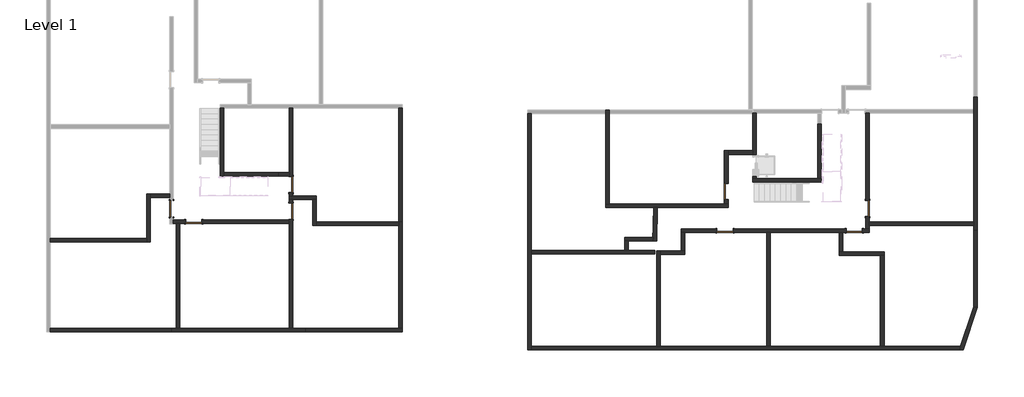
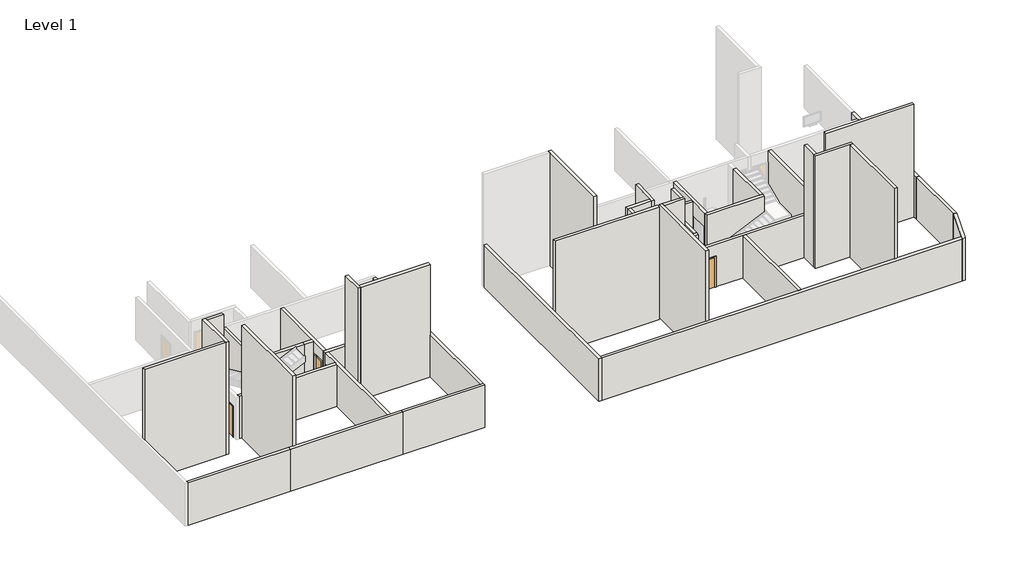
# One storey, part 1 of 2: 44 walls, 8 doors.
"""IFC4 building model written with IfcOpenShell, lengths in millimetres."""

import ifcopenshell
import ifcopenshell.guid

model = None  # the IFC model being written
_history = None  # IfcOwnerHistory: only IFC2X3 demands one
_inside = {}  # id of a spatial element -> (the spatial element, [elements in it])
_under = {}  # id of a project, library or spatial element -> (it, [spatial elements below it])
_declared = {}  # id of a project -> (the project, [libraries it declares])
_typed = {}  # id of a type object -> (the type object, [elements of that type])
_made_of = {}  # id of a material, layer set ... -> (it, [elements and type objects made of it])


def new_model(schema):
    """Start an empty IFC model of exactly this schema.

    Asked for "IFC4X3", IfcOpenShell would pick the latest addendum, in which some entities
    have other attributes; the version numbers below select the first issue.
    IFC2X3 requires an IfcOwnerHistory on every rooted entity: one is made here for all.
    """
    global model, _history
    if schema == "IFC4X3":
        model = ifcopenshell.file(schema_version=(4, 3, 0, 0))
    else:
        model = ifcopenshell.file(schema=schema)
    _inside.clear()
    _under.clear()
    _declared.clear()
    _typed.clear()
    _made_of.clear()
    _history = None
    if model.schema == "IFC2X3":
        org = make("IfcOrganization", Name="unknown")
        user = make(
            "IfcPersonAndOrganization",
            ThePerson=make("IfcPerson", FamilyName="unknown"),
            TheOrganization=org,
        )
        app = make(
            "IfcApplication",
            ApplicationDeveloper=org,
            Version="unknown",
            ApplicationFullName="unknown",
            ApplicationIdentifier="unknown",
        )
        _history = make(
            "IfcOwnerHistory",
            OwningUser=user,
            OwningApplication=app,
            ChangeAction="ADDED",
            CreationDate=0,
        )
    return model


def make(cls, **values):
    """One entity of the class cls with the attributes given. An attribute that is None is left unset."""
    return model.create_entity(
        cls, **{name: value for name, value in values.items() if value is not None}
    )


def rooted(cls, **values):
    """An entity with a GlobalId (a new one), such as an element, a storey or a relation."""
    return make(cls, GlobalId=ifcopenshell.guid.new(), OwnerHistory=_history, **values)


def si_unit(unit_type, name, prefix=None):
    """IfcSIUnit, for example si_unit("LENGTHUNIT", "METRE", prefix="MILLI")."""
    return make("IfcSIUnit", UnitType=unit_type, Prefix=prefix, Name=name)


def assignment(units):
    """IfcUnitAssignment: the units of a project."""
    return None if units is None else make("IfcUnitAssignment", Units=units)


def point(xyz):
    """IfcCartesianPoint."""
    return None if xyz is None else make("IfcCartesianPoint", Coordinates=xyz)


def direction(xyz):
    """IfcDirection."""
    return None if xyz is None else make("IfcDirection", DirectionRatios=xyz)


def frame(location, z_axis=None, x_axis=None):
    """IfcAxis2Placement3D, a coordinate frame: its origin and axes. An axis left out is left unset."""
    return make(
        "IfcAxis2Placement3D",
        Location=point(location),
        Axis=direction(z_axis),
        RefDirection=direction(x_axis),
    )


def origin():
    """The frame at (0, 0, 0) with its axes left unset."""
    return frame((0.0, 0.0, 0.0))


def origin_with_axes():
    """The frame at (0, 0, 0) with the z axis (0, 0, 1) and the x axis (1, 0, 0) written out."""
    return frame((0.0, 0.0, 0.0), z_axis=(0.0, 0.0, 1.0), x_axis=(1.0, 0.0, 0.0))


def place(relative_to, where):
    """IfcLocalPlacement: puts the frame where relative to a parent placement (None: the world)."""
    return make(
        "IfcLocalPlacement", PlacementRelTo=relative_to, RelativePlacement=where
    )


def context(
    kind, dimensions, precision=None, world=None, true_north=None, identifier=None
):
    """IfcGeometricRepresentationContext, for example the 3D "Model" context."""
    return make(
        "IfcGeometricRepresentationContext",
        ContextIdentifier=identifier,
        ContextType=kind,
        CoordinateSpaceDimension=dimensions,
        Precision=precision,
        WorldCoordinateSystem=world,
        TrueNorth=true_north,
    )


def project(units=None, contexts=None):
    """IfcProject with its units and contexts."""
    return rooted(
        "IfcProject",
        Name="project",
        RepresentationContexts=contexts,
        UnitsInContext=assignment(units),
    )


def spatial(cls, under=None, at=None, **own):
    """A site, building, storey or space (cls), placed at a placement, below another one or the project."""
    s = rooted(cls, ObjectPlacement=at, **own)
    if under is not None:
        _under.setdefault(under.id(), (under, []))[1].append(s)
    return s


def polyline(points):
    """IfcPolyline through the points."""
    return make("IfcPolyline", Points=[point(p) for p in points])


def outline(outer, holes=None, kind="AREA"):
    """IfcArbitraryClosedProfileDef: a profile drawn as a closed curve; with holes, ...WithVoids."""
    if holes is None:
        return make("IfcArbitraryClosedProfileDef", ProfileType=kind, OuterCurve=outer)
    return make(
        "IfcArbitraryProfileDefWithVoids",
        ProfileType=kind,
        OuterCurve=outer,
        InnerCurves=holes,
    )


def extrude(swept, where, along, depth):
    """IfcExtrudedAreaSolid: the profile swept, set in the frame where, extruded along a direction by depth."""
    return make(
        "IfcExtrudedAreaSolid",
        SweptArea=swept,
        Position=where,
        ExtrudedDirection=direction(along),
        Depth=depth,
    )


def faces_of(points, faces, orient=None, outer=None):
    """IfcFace entities. A face is a list of loops; a loop is a list of indices into points, from 0.

    orient and outer hold one flag for each loop. By default every Orientation is true, the
    first loop of a face is its IfcFaceOuterBound and the others are IfcFaceBound.
    """
    made = []
    for i, loops in enumerate(faces):
        bounds = []
        for j, loop in enumerate(loops):
            is_outer = j == 0 if outer is None else outer[i][j]
            bounds.append(
                make(
                    "IfcFaceOuterBound" if is_outer else "IfcFaceBound",
                    Bound=make("IfcPolyLoop", Polygon=[points[k] for k in loop]),
                    Orientation=True if orient is None else orient[i][j],
                )
            )
        made.append(make("IfcFace", Bounds=bounds))
    return made


def faceted_brep(points, faces, orient=None, outer=None, voids=None):
    """IfcFacetedBrep: a solid bounded by flat faces; with voids (closed shells), ...WithVoids."""
    shared = [point(p) for p in points]
    hull = make("IfcClosedShell", CfsFaces=faces_of(shared, faces, orient, outer))
    if voids is None:
        return make("IfcFacetedBrep", Outer=hull)
    return make(
        "IfcFacetedBrepWithVoids",
        Outer=hull,
        Voids=[
            make(cls, CfsFaces=faces_of(shared, fs, o, b)) for cls, fs, o, b in voids
        ],
    )


def shape(context_of_items, identifier, shape_type, items):
    """IfcShapeRepresentation: the items that make up one representation, for example the "Body"."""
    return make(
        "IfcShapeRepresentation",
        ContextOfItems=context_of_items,
        RepresentationIdentifier=identifier,
        RepresentationType=shape_type,
        Items=items,
    )


def source(mapping_origin, context_of_items, identifier, shape_type, items):
    """IfcRepresentationMap: a shape defined once, which mapped items show again and again."""
    return make(
        "IfcRepresentationMap",
        MappingOrigin=mapping_origin,
        MappedRepresentation=shape(context_of_items, identifier, shape_type, items),
    )


def transform(
    local_origin,
    x_axis=None,
    y_axis=None,
    z_axis=None,
    scale=None,
    scale2=None,
    scale3=None,
    uniform=True,
):
    """IfcCartesianTransformationOperator3D, or its non-uniform kind. x_axis, y_axis, z_axis: its Axis1, 2, 3."""
    if uniform:
        return make(
            "IfcCartesianTransformationOperator3D",
            Axis1=direction(x_axis),
            Axis2=direction(y_axis),
            LocalOrigin=point(local_origin),
            Scale=scale,
            Axis3=direction(z_axis),
        )
    return make(
        "IfcCartesianTransformationOperator3DnonUniform",
        Axis1=direction(x_axis),
        Axis2=direction(y_axis),
        LocalOrigin=point(local_origin),
        Scale=scale,
        Axis3=direction(z_axis),
        Scale2=scale2,
        Scale3=scale3,
    )


def mapped(mapping_source, mapping_target):
    """IfcMappedItem: shows the shape of a source again, moved by a transform."""
    return make(
        "IfcMappedItem", MappingSource=mapping_source, MappingTarget=mapping_target
    )


def made_of(thing, what):
    """Note that an element or type object is made of a material, layer set ...; save() writes the relation."""
    if what is not None:
        _made_of.setdefault(what.id(), (what, []))[1].append(thing)
    return thing


def element(
    cls,
    number,
    at=None,
    inside=None,
    cuts=None,
    type_object=None,
    material=None,
    context=None,
    identifier="Body",
    shape_type=None,
    held_by="IfcProductDefinitionShape",
    body=None,
    shapes=None,
    **own,
):
    """One element of the class cls, such as IfcWall. Its Tag is "e" and its number.

    at: its placement. inside: the storey or other place that contains it. cuts: it is an
    opening in that element (IfcRelVoidsElement). A single representation is given by context,
    identifier, shape_type and body (its items); several are given by shapes. held_by: the class
    of the entity that holds the representations. save() writes the other relations.
    """
    e = rooted(cls, Tag="e%d" % number, ObjectPlacement=at, **own)
    if body is not None:
        shapes = [shape(context, identifier, shape_type, body)]
    if shapes is not None:
        e.Representation = make(held_by, Representations=shapes)
    if inside is not None:
        _inside.setdefault(inside.id(), (inside, []))[1].append(e)
    if cuts is not None:
        rooted(
            "IfcRelVoidsElement", RelatingBuildingElement=cuts, RelatedOpeningElement=e
        )
    if type_object is not None:
        _typed.setdefault(type_object.id(), (type_object, []))[1].append(e)
    return made_of(e, material)


def aggregate(whole, parts):
    """IfcRelAggregates: a whole, such as a stair, and the parts it consists of."""
    return rooted("IfcRelAggregates", RelatingObject=whole, RelatedObjects=parts)


def save(model, path):
    """Write the relations noted so far, then the file.

    IfcRelAggregates (storeys below a building ...), IfcRelContainedInSpatialStructure (elements
    in a storey), IfcRelDefinesByType, IfcRelAssociatesMaterial and IfcRelDeclares: one each for
    every whole, place, type object, material and project.
    """
    for whole, parts in _under.values():
        aggregate(whole, parts)
    for where, things in _inside.values():
        rooted(
            "IfcRelContainedInSpatialStructure",
            RelatedElements=things,
            RelatingStructure=where,
        )
    for kind, things in _typed.values():
        rooted("IfcRelDefinesByType", RelatedObjects=things, RelatingType=kind)
    for what, things in _made_of.values():
        rooted("IfcRelAssociatesMaterial", RelatedObjects=things, RelatingMaterial=what)
    for by, libraries in _declared.values():
        rooted("IfcRelDeclares", RelatingContext=by, RelatedDefinitions=libraries)
    model.write(path)


def m_single_flush_0915_x_2134mm_727434cd(model_context):
    return source(origin(), model_context, "Body", "SweptSolid", [
        extrude(outline(polyline([(2210.0, -533.5), (0.0, -533.5), (0.0, -457.5), (2134.0, -457.5), (2134.0, 457.5), (0.0, 457.5), (0.0, 533.5), (2210.0, 533.5), (2210.0, -533.5)])), frame((0.0, -125.0, 0.0), z_axis=(0.0, 1.0, 0.0), x_axis=(0.0, 0.0, 1.0)), (0.0, 0.0, 1.0), 25.0),
        extrude(outline(polyline([(2210.0, 533.5), (2210.0, -533.5), (0.0, -533.5), (0.0, -457.5), (2134.0, -457.5), (2134.0, 457.5), (0.0, 457.5), (0.0, 533.5), (2210.0, 533.5)])), frame((0.0, 100.0, 0.0), z_axis=(0.0, 1.0, 0.0), x_axis=(0.0, 0.0, 1.0)), (0.0, 0.0, 1.0), 25.0),
        extrude(outline(polyline([(457.5, -49.0), (457.5, -100.0), (-457.5, -100.0), (-457.5, -49.0), (457.5, -49.0)])), origin_with_axes(), (0.0, 0.0, 1.0), 2134.0),
    ])


def m_single_flush_0915_x_2134mm_6a9e8738(model_context):
    return source(origin(), model_context, "Body", "SweptSolid", [
        extrude(outline(polyline([(2210.0, -533.5), (0.0, -533.5), (0.0, -457.5), (2134.0, -457.5), (2134.0, 457.5), (0.0, 457.5), (0.0, 533.5), (2210.0, 533.5), (2210.0, -533.5)])), frame((0.0, 100.0, 0.0), z_axis=(0.0, 1.0, 0.0), x_axis=(0.0, 0.0, 1.0)), (0.0, 0.0, 1.0), 25.0),
        extrude(outline(polyline([(2210.0, 533.5), (2210.0, -533.5), (0.0, -533.5), (0.0, -457.5), (2134.0, -457.5), (2134.0, 457.5), (0.0, 457.5), (0.0, 533.5), (2210.0, 533.5)])), frame((0.0, -125.0, 0.0), z_axis=(0.0, 1.0, 0.0), x_axis=(0.0, 0.0, 1.0)), (0.0, 0.0, 1.0), 25.0),
        extrude(outline(polyline([(457.5, 49.0), (-457.5, 49.0), (-457.5, 100.0), (457.5, 100.0), (457.5, 49.0)])), origin_with_axes(), (0.0, 0.0, 1.0), 2134.0),
    ])


model = new_model("IFC4")

# Units and contexts
model_context = context("Model", 3, world=origin())
ifc_project = project(units=[si_unit("LENGTHUNIT", "METRE", prefix="MILLI")], contexts=[model_context])

# Site, building, storey
site = spatial("IfcSite", under=ifc_project)
building = spatial("IfcBuilding", under=site)
storey = spatial("IfcBuildingStorey", under=building, Name="Level 1", Elevation=0.0)

# Doors
placement = place(None, origin())
m_single_flush_0915_x_2134mm_shape = m_single_flush_0915_x_2134mm_727434cd(model_context)
element("IfcDoor", 1, ObjectType="M_Single-Flush : 0915 x 2134mm", at=placement, inside=storey, context=model_context, shape_type="MappedRepresentation", body=[
    mapped(m_single_flush_0915_x_2134mm_shape, transform((16070.6041014, -3023.024372, 0.0), x_axis=(0.0, -1.0, 0.0), y_axis=(1.0, 0.0, 0.0), z_axis=(0.0, 0.0, 1.0))),
])
element("IfcDoor", 2, ObjectType="M_Single-Flush : 0915 x 2134mm", at=placement, inside=storey, context=model_context, shape_type="MappedRepresentation", body=[
    mapped(m_single_flush_0915_x_2134mm_shape, transform((16002.336337, -5240.0098119, 0.0), x_axis=(1.0, 0.0, 0.0), y_axis=(0.0, 1.0, 0.0), z_axis=(0.0, 0.0, 1.0))),
])
element("IfcDoor", 3, ObjectType="M_Single-Flush : 0915 x 2134mm", at=placement, inside=storey, context=model_context, shape_type="MappedRepresentation", body=[
    mapped(m_single_flush_0915_x_2134mm_shape, transform((-8530.3449834, -4137.6378151, 0.0), x_axis=(0.0, 1.0, 0.0), y_axis=(-1.0, 0.0, 0.0), z_axis=(0.0, 0.0, 1.0))),
])
m_single_flush_0915_x_2134mm_2_shape = m_single_flush_0915_x_2134mm_6a9e8738(model_context)
element("IfcDoor", 4, ObjectType="M_Single-Flush : 0915 x 2134mm", at=placement, inside=storey, context=model_context, shape_type="MappedRepresentation", body=[
    mapped(m_single_flush_0915_x_2134mm_2_shape, transform((24048.8612349, -3982.5098119, 0.0), x_axis=(0.0, -1.0, 0.0), y_axis=(1.0, 0.0, 0.0), z_axis=(0.0, 0.0, 1.0))),
])
element("IfcDoor", 5, ObjectType="M_Single-Flush : 0915 x 2134mm", at=placement, inside=storey, context=model_context, shape_type="MappedRepresentation", body=[
    mapped(m_single_flush_0915_x_2134mm_2_shape, transform((23308.8612349, -5240.0098119, 0.0), x_axis=(-1.0, 0.0, 0.0), y_axis=(0.0, -1.0, 0.0), z_axis=(0.0, 0.0, 1.0))),
])
element("IfcDoor", 6, ObjectType="M_Single-Flush : 0915 x 2134mm", at=placement, inside=storey, context=model_context, shape_type="MappedRepresentation", body=[
    mapped(m_single_flush_0915_x_2134mm_2_shape, transform((-14032.3304233, -4739.1627129, 0.0), x_axis=(-1.0, 0.0, 0.0), y_axis=(0.0, -1.0, 0.0), z_axis=(0.0, 0.0, 1.0))),
])
element("IfcDoor", 7, ObjectType="M_Single-Flush : 0915 x 2134mm", at=placement, inside=storey, context=model_context, shape_type="MappedRepresentation", body=[
    mapped(m_single_flush_0915_x_2134mm_2_shape, transform((-8530.3449834, -2622.6378151, 0.0), x_axis=(0.0, -1.0, 0.0), y_axis=(1.0, 0.0, 0.0), z_axis=(0.0, 0.0, 1.0))),
])
element("IfcDoor", 8, ObjectType="M_Single-Flush : 0915 x 2134mm", at=placement, inside=storey, context=model_context, shape_type="MappedRepresentation", body=[
    mapped(m_single_flush_0915_x_2134mm_2_shape, transform((-15289.8304233, -3999.1627129, 0.0), x_axis=(0.0, 1.0, 0.0), y_axis=(-1.0, 0.0, 0.0), z_axis=(0.0, 0.0, 1.0))),
])

# Walls
element("IfcWall", 9, ObjectType="Generic - 200mm", at=placement, inside=storey, context=model_context, shape_type="Brep", body=[
    faceted_brep([(30068.8612349, 2319.475628, 0.0), (30068.8612349, 1619.475628, 0.0), (30068.8612349, 1419.475628, 0.0), (30068.8612349, -4760.0098119, 0.0), (30068.8612349, -4960.0098119, 0.0), (30068.8612349, -5240.0098119, 0.0), (30068.8612349, -5240.0098119, 3000.0), (30068.8612349, 1419.475628, 3000.0), (30068.8612349, 1619.475628, 3000.0), (30068.8612349, 2319.475628, 3000.0), (30268.8612349, 2319.475628, 0.0), (30268.8612349, 2319.475628, 3000.0), (30268.8612349, -5240.0098119, 3000.0), (30268.8612349, -5240.0098119, 0.0), (30268.3425199, 2319.475628, 0.0), (30069.3799498, -5240.0098119, 0.0), (30069.3799498, -5240.0098119, 3000.0), (30268.3425199, 2319.475628, 3000.0)], [[[0, 1, 2, 3, 4, 5, 6, 7, 8, 9]], [[10, 11, 12, 13]], [[5, 4, 3, 2, 1, 0, 14, 10, 13, 15]], [[6, 5, 15, 13, 12, 16]], [[9, 8, 7, 6, 16, 12, 11, 17]], [[0, 9, 17, 11, 10, 14]]]),
])
element("IfcWall", 10, ObjectType="Generic - 200mm", at=placement, inside=storey, context=model_context, shape_type="Brep", body=[
    faceted_brep([(30069.3799498, -5240.0098119, 0.0), (30069.3799498, -9543.0251929, 0.0), (30069.3799498, -9543.0251929, 3000.0), (30069.3799498, -5240.0098119, 3000.0), (30269.3799498, -5240.0098119, 0.0), (30269.3799498, -5240.0098119, 3000.0), (30269.3799498, -9575.863443, 3000.0), (30269.3799498, -9575.863443, 0.0), (30268.8612349, -5240.0098119, 0.0), (30268.8612349, -5240.0098119, 3000.0)], [[[0, 1, 2, 3]], [[4, 5, 6, 7]], [[1, 0, 8, 4, 7]], [[3, 2, 6, 5, 9]], [[0, 3, 9, 5, 4, 8]], [[2, 1, 7, 6]]]),
])
element("IfcWall", 11, ObjectType="Generic - 200mm", at=placement, inside=storey, context=model_context, shape_type="Brep", body=[
    faceted_brep([(21449.836337, -2276.2808257, 0.0), (21249.836337, -2276.2808257, 0.0), (17770.6041014, -2276.2808257, 0.0), (17570.6041014, -2276.2808257, 0.0), (17570.6041014, -2276.2808257, 3000.0), (17770.6041014, -2276.2808257, 3000.0), (21249.836337, -2276.2808257, 3000.0), (21449.836337, -2276.2808257, 3000.0), (21449.836337, -2476.2808257, 0.0), (21449.836337, -2476.2808257, 3000.0), (17570.6041014, -2476.2808257, 3000.0), (17570.6041014, -2476.2808257, 0.0)], [[[0, 1, 2, 3, 4, 5, 6, 7]], [[8, 9, 10, 11]], [[3, 2, 1, 0, 8, 11]], [[7, 6, 5, 4, 10, 9]], [[0, 7, 9, 8]], [[4, 3, 11, 10]]]),
])
element("IfcWall", 12, ObjectType="Generic - 200mm", at=placement, inside=storey, context=model_context, shape_type="SweptSolid", body=[
    extrude(outline(polyline([(18559.836337, -5340.0098119), (18559.836337, -11796.6907835), (18359.836337, -11796.6907835), (18359.836337, -5340.0098119), (18559.836337, -5340.0098119)])), origin_with_axes(), (0.0, 0.0, 1.0), 3000.0),
])
element("IfcWall", 13, ObjectType="Generic - 200mm", at=placement, inside=storey, context=model_context, shape_type="Brep", body=[
    faceted_brep([(29308.8116245, -11796.6907835, 0.0), (24988.8612349, -11796.6907835, 0.0), (24788.8612349, -11796.6907835, 0.0), (18559.836337, -11796.6907835, 0.0), (18359.836337, -11796.6907835, 0.0), (12342.1281129, -11796.6907835, 0.0), (12142.1281129, -11796.6907835, 0.0), (5043.716007, -11796.6907835, 0.0), (5043.716007, -11796.6907835, 3000.0), (18359.836337, -11796.6907835, 3000.0), (18559.836337, -11796.6907835, 3000.0), (29308.8116245, -11796.6907835, 3000.0), (29241.3155126, -11996.6907835, 0.0), (29241.3155126, -11996.6907835, 3000.0), (5043.716007, -11996.6907835, 3000.0), (5043.716007, -11996.6907835, 0.0)], [[[0, 1, 2, 3, 4, 5, 6, 7, 8, 9, 10, 11]], [[12, 13, 14, 15]], [[7, 6, 5, 4, 3, 2, 1, 0, 12, 15]], [[11, 10, 9, 8, 14, 13]], [[0, 11, 13, 12]], [[8, 7, 15, 14]]]),
])
element("IfcWall", 14, ObjectType="Generic - 200mm", at=placement, inside=storey, context=model_context, shape_type="Brep", body=[
    faceted_brep([(30069.3799498, -9543.0251929, 0.0), (29308.8116245, -11796.6907835, 0.0), (29241.3155126, -11996.6907835, 0.0), (29241.3155126, -11996.6907835, 3000.0), (29308.8116245, -11796.6907835, 3000.0), (30069.3799498, -9543.0251929, 3000.0), (30269.3799498, -9575.863443, 0.0), (30269.3799498, -9575.863443, 3000.0), (29452.3977836, -11996.6907835, 3000.0), (29452.3977836, -11996.6907835, 0.0)], [[[0, 1, 2, 3, 4, 5]], [[6, 7, 8, 9]], [[2, 1, 0, 6, 9]], [[5, 4, 3, 8, 7]], [[0, 5, 7, 6]], [[3, 2, 9, 8]]]),
])
element("IfcWall", 15, ObjectType="Generic - 200mm", at=placement, inside=storey, context=model_context, shape_type="Brep", body=[
    faceted_brep([(22851.3612349, -5140.0098119, 2134.0), (22851.3612349, -5140.0098119, 0.0), (16459.836337, -5140.0098119, 0.0), (16459.836337, -5140.0098119, 2134.0), (15544.836337, -5140.0098119, 2134.0), (15544.836337, -5140.0098119, 0.0), (13532.1281129, -5140.0098119, 0.0), (13532.1281129, -5140.0098119, 3000.0), (23948.8612349, -5140.0098119, 3000.0), (24148.8612349, -5140.0098119, 3000.0), (24163.3998354, -5140.0098119, 3000.0), (24163.3998354, -5140.0098119, 0.0), (24148.8612349, -5140.0098119, 0.0), (23948.8612349, -5140.0098119, 0.0), (23766.3612349, -5140.0098119, 0.0), (23766.3612349, -5140.0098119, 2134.0), (16459.836337, -5340.0098119, 0.0), (18359.836337, -5340.0098119, 0.0), (18559.836337, -5340.0098119, 0.0), (22468.8612349, -5340.0098119, 0.0), (22668.8612349, -5340.0098119, 0.0), (22851.3612349, -5340.0098119, 0.0), (22851.3612349, -5340.0098119, 2134.0), (23766.3612349, -5340.0098119, 2134.0), (23766.3612349, -5340.0098119, 0.0), (24163.3998354, -5340.0098119, 0.0), (24163.3998354, -5340.0098119, 3000.0), (18559.836337, -5340.0098119, 3000.0), (18359.836337, -5340.0098119, 3000.0), (13532.1281129, -5340.0098119, 3000.0), (13532.1281129, -5340.0098119, 0.0), (13732.1281129, -5340.0098119, 0.0), (15544.836337, -5340.0098119, 0.0), (15544.836337, -5340.0098119, 2134.0), (16459.836337, -5340.0098119, 2134.0)], [[[0, 1, 2, 3, 4, 5, 6, 7, 8, 9, 10, 11, 12, 13, 14, 15]], [[16, 17, 18, 19, 20, 21, 22, 23, 24, 25, 26, 27, 28, 29, 30, 31, 32, 33, 34]], [[2, 1, 21, 20, 19, 18, 17, 16]], [[14, 13, 12, 11, 25, 24]], [[30, 6, 5, 32, 31]], [[10, 9, 8, 7, 29, 28, 27, 26]], [[11, 10, 26, 25]], [[34, 3, 2, 16]], [[4, 33, 32, 5]], [[33, 4, 3, 34]], [[22, 21, 1, 0]], [[23, 22, 0, 15]], [[24, 23, 15, 14]], [[7, 6, 30, 29]]]),
])
element("IfcWall", 16, ObjectType="Generic - 200mm", at=placement, inside=storey, context=model_context, shape_type="Brep", body=[
    faceted_brep([(4843.716007, 1379.9901881, 0.0), (4843.716007, -11996.6907835, 0.0), (4843.716007, -11996.6907835, 3000.0), (4843.716007, 1379.9901881, 3000.0), (5043.716007, 1379.9901881, 0.0), (5043.716007, 1379.9901881, 3000.0), (5043.716007, -11796.6907835, 3000.0), (5043.716007, -11996.6907835, 3000.0), (5043.716007, -11996.6907835, 0.0), (5043.716007, -11796.6907835, 0.0), (5043.716007, -6560.0098119, 0.0), (5043.716007, -6360.0098119, 0.0)], [[[0, 1, 2, 3]], [[4, 5, 6, 7, 8, 9, 10, 11]], [[1, 0, 4, 11, 10, 9, 8]], [[3, 2, 7, 6, 5]], [[2, 1, 8, 7]], [[0, 3, 5, 4]]]),
])
element("IfcWall", 17, ObjectType="Generic - 200mm", at=placement, inside=storey, context=model_context, shape_type="Brep", body=[
    faceted_brep([(24148.8612349, 1419.475628, 3000.0), (24148.8612349, -5140.0098119, 3000.0), (24148.8612349, -5140.0098119, 0.0), (24148.8612349, -4960.0098119, 0.0), (24148.8612349, -4760.0098119, 0.0), (24148.8612349, -4440.0098119, 0.0), (24148.8612349, -4440.0098119, 2134.0), (24148.8612349, -3525.0098119, 2134.0), (24148.8612349, -3525.0098119, 0.0), (24148.8612349, 1419.475628, 0.0), (23948.8612349, -5140.0098119, 3000.0), (23948.8612349, 1419.475628, 3000.0), (23948.8612349, 1419.475628, 0.0), (23948.8612349, -3525.0098119, 0.0), (23948.8612349, -3525.0098119, 2134.0), (23948.8612349, -4440.0098119, 2134.0), (23948.8612349, -4440.0098119, 0.0), (23948.8612349, -5140.0098119, 0.0)], [[[0, 1, 2, 3, 4, 5, 6, 7, 8, 9]], [[10, 11, 12, 13, 14, 15, 16, 17]], [[12, 9, 8, 13]], [[2, 17, 16, 5, 4, 3]], [[1, 0, 11, 10]], [[0, 9, 12, 11]], [[15, 6, 5, 16]], [[7, 14, 13, 8]], [[14, 7, 6, 15]], [[2, 1, 10, 17]]]),
])
element("IfcWall", 18, ObjectType="Generic - 200mm", at=placement, inside=storey, context=model_context, shape_type="SweptSolid", body=[
    extrude(outline(polyline([(21249.836337, -2276.2808257), (21249.836337, 799.475628), (21449.836337, 799.475628), (21449.836337, -2276.2808257), (21249.836337, -2276.2808257)])), origin_with_axes(), (0.0, 0.0, 1.0), 3000.0),
])
element("IfcWall", 19, ObjectType="Generic - 200mm", at=placement, inside=storey, context=model_context, shape_type="Brep", body=[
    faceted_brep([(17570.6041014, -2276.2808257, 3000.0), (17570.6041014, -920.524372, 3000.0), (17570.6041014, -720.524372, 3000.0), (17570.6041014, 1379.475628, 3000.0), (17570.6041014, 1419.475628, 3000.0), (17570.6041014, 1419.475628, 0.0), (17570.6041014, 1379.475628, 0.0), (17570.6041014, -720.524372, 0.0), (17570.6041014, -920.524372, 0.0), (17570.6041014, -926.2808257, 0.0), (17570.6041014, -926.2808257, 2000.0), (17570.6041014, -2181.2876228, 2000.0), (17570.6041014, -2181.2876228, 0.0), (17570.6041014, -2276.2808257, 0.0), (17770.6041014, 1419.475628, 3000.0), (17770.6041014, -2276.2808257, 3000.0), (17770.6041014, -2276.2808257, 0.0), (17770.6041014, -2181.2876228, 0.0), (17770.6041014, -2181.2876228, 2000.0), (17770.6041014, -926.2808257, 2000.0), (17770.6041014, -926.2808257, 0.0), (17770.6041014, 1419.475628, 0.0)], [[[0, 1, 2, 3, 4, 5, 6, 7, 8, 9, 10, 11, 12, 13]], [[14, 15, 16, 17, 18, 19, 20, 21]], [[16, 13, 12, 17]], [[5, 21, 20, 9, 8, 7, 6]], [[4, 3, 2, 1, 0, 15, 14]], [[0, 13, 16, 15]], [[5, 4, 14, 21]], [[11, 18, 17, 12]], [[19, 10, 9, 20]], [[10, 19, 18, 11]]]),
])
element("IfcWall", 20, ObjectType="Generic - 200mm", at=placement, inside=storey, context=model_context, shape_type="Brep", body=[
    faceted_brep([(9268.8612349, -3940.0098119, 0.0), (11970.0065607, -3940.0098119, 0.0), (12170.0511873, -3940.0098119, 0.0), (16170.6041014, -3940.0098119, 0.0), (16170.6041014, -3940.0098119, 3000.0), (9268.8612349, -3940.0098119, 3000.0), (9268.8612349, -3740.0098119, 0.0), (9268.8612349, -3740.0098119, 3000.0), (15970.6041014, -3740.0098119, 3000.0), (16170.6041014, -3740.0098119, 3000.0), (16170.6041014, -3740.0098119, 0.0), (15970.6041014, -3740.0098119, 0.0), (9468.8612349, -3740.0098119, 0.0)], [[[0, 1, 2, 3, 4, 5]], [[6, 7, 8, 9, 10, 11, 12]], [[3, 2, 1, 0, 6, 12, 11, 10]], [[5, 4, 9, 8, 7]], [[4, 3, 10, 9]], [[0, 5, 7, 6]]]),
])
element("IfcWall", 21, ObjectType="Generic - 200mm", at=placement, inside=storey, context=model_context, shape_type="Brep", body=[
    faceted_brep([(16170.6041014, -720.524372, 3000.0), (16170.6041014, -920.524372, 3000.0), (16170.6041014, -3740.0098119, 3000.0), (16170.6041014, -3740.0098119, 0.0), (16170.6041014, -3480.524372, 0.0), (16170.6041014, -3480.524372, 2134.0), (16170.6041014, -2565.524372, 2134.0), (16170.6041014, -2565.524372, 0.0), (16170.6041014, -920.524372, 0.0), (16170.6041014, -720.524372, 0.0), (15970.6041014, -3740.0098119, 3000.0), (15970.6041014, -720.524372, 3000.0), (15970.6041014, -720.524372, 0.0), (15970.6041014, -2565.524372, 0.0), (15970.6041014, -2565.524372, 2134.0), (15970.6041014, -3480.524372, 2134.0), (15970.6041014, -3480.524372, 0.0), (15970.6041014, -3740.0098119, 0.0)], [[[0, 1, 2, 3, 4, 5, 6, 7, 8, 9]], [[10, 11, 12, 13, 14, 15, 16, 17]], [[3, 17, 16, 4]], [[12, 9, 8, 7, 13]], [[2, 1, 0, 11, 10]], [[3, 2, 10, 17]], [[0, 9, 12, 11]], [[15, 5, 4, 16]], [[6, 14, 13, 7]], [[14, 6, 5, 15]]]),
])
element("IfcWall", 22, ObjectType="Generic - 200mm", at=placement, inside=storey, context=model_context, shape_type="SweptSolid", body=[
    extrude(outline(polyline([(17570.6041014, -920.524372), (16170.6041014, -920.524372), (16170.6041014, -720.524372), (17570.6041014, -720.524372), (17570.6041014, -920.524372)])), origin_with_axes(), (0.0, 0.0, 1.0), 3000.0),
])
element("IfcWall", 23, ObjectType="Generic - 200mm", at=placement, inside=storey, context=model_context, shape_type="Brep", body=[
    faceted_brep([(22468.8612349, -6641.2808257, 0.0), (24788.8612349, -6641.2808257, 0.0), (24988.8612349, -6641.2808257, 0.0), (24988.8612349, -6641.2808257, 8000.0), (24788.8612349, -6641.2808257, 8000.0), (22468.8612349, -6641.2808257, 8000.0), (22468.8612349, -6441.2808257, 0.0), (22468.8612349, -6441.2808257, 8000.0), (22668.8612349, -6441.2808257, 8000.0), (24988.8612349, -6441.2808257, 8000.0), (24988.8612349, -6441.2808257, 0.0), (22668.8612349, -6441.2808257, 0.0)], [[[0, 1, 2, 3, 4, 5]], [[6, 7, 8, 9, 10, 11]], [[2, 1, 0, 6, 11, 10]], [[5, 4, 3, 9, 8, 7]], [[3, 2, 10, 9]], [[0, 5, 7, 6]]]),
])
element("IfcWall", 24, ObjectType="Generic - 200mm", at=placement, inside=storey, context=model_context, shape_type="SweptSolid", body=[
    extrude(outline(polyline([(24788.8612349, -11796.6907835), (24788.8612349, -6641.2808257), (24988.8612349, -6641.2808257), (24988.8612349, -11796.6907835), (24788.8612349, -11796.6907835)])), origin_with_axes(), (0.0, 0.0, 1.0), 8000.0),
])
element("IfcWall", 25, ObjectType="Generic - 200mm", at=placement, inside=storey, context=model_context, shape_type="SweptSolid", body=[
    extrude(outline(polyline([(22668.8612349, -5340.0098119), (22668.8612349, -6441.2808257), (22468.8612349, -6441.2808257), (22468.8612349, -5340.0098119), (22668.8612349, -5340.0098119)])), origin_with_axes(), (0.0, 0.0, 1.0), 8000.0),
])
element("IfcWall", 26, ObjectType="Generic - 200mm", at=placement, inside=storey, context=model_context, shape_type="SweptSolid", body=[
    extrude(outline(polyline([(30068.8612349, -4960.0098119), (24148.8612349, -4960.0098119), (24148.8612349, -4760.0098119), (30068.8612349, -4760.0098119), (30068.8612349, -4960.0098119)])), origin_with_axes(), (0.0, 0.0, 1.0), 8000.0),
])
element("IfcWall", 27, ObjectType="Generic - 200mm", at=placement, inside=storey, context=model_context, shape_type="Brep", body=[
    faceted_brep([(9268.8612349, 1579.9901881, 0.0), (9268.8612349, 1379.9901881, 0.0), (9268.8612349, -3740.0098119, 0.0), (9268.8612349, -3740.0098119, 3000.0), (9268.8612349, -3740.0098119, 8000.0), (9268.8612349, 1379.9901881, 8000.0), (9268.8612349, 1579.9901881, 8000.0), (9468.8612349, 1579.9901881, 0.0), (9468.8612349, 1579.9901881, 8000.0), (9468.8612349, -3740.0098119, 8000.0), (9468.8612349, -3740.0098119, 0.0), (9468.8612349, 1379.475628, 0.0), (9468.8612349, 1579.475628, 0.0)], [[[0, 1, 2, 3, 4, 5, 6]], [[7, 8, 9, 10, 11, 12]], [[2, 1, 0, 7, 12, 11, 10]], [[6, 5, 4, 9, 8]], [[4, 3, 2, 10, 9]], [[0, 6, 8, 7]]]),
])
element("IfcWall", 28, ObjectType="Generic - 200mm", at=placement, inside=storey, context=model_context, shape_type="Brep", body=[
    faceted_brep([(12016.7908757, -6360.0098119, 0.0), (10530.3209687, -6360.0098119, 0.0), (10330.3209687, -6360.0098119, 0.0), (5043.716007, -6360.0098119, 0.0), (5043.716007, -6360.0098119, 8000.0), (10330.3209687, -6360.0098119, 8000.0), (10530.3209687, -6360.0098119, 8000.0), (12016.7908757, -6360.0098119, 8000.0), (12016.7908757, -6560.0098119, 0.0), (12016.7908757, -6560.0098119, 8000.0), (5043.716007, -6560.0098119, 8000.0), (5043.716007, -6560.0098119, 0.0)], [[[0, 1, 2, 3, 4, 5, 6, 7]], [[8, 9, 10, 11]], [[3, 2, 1, 0, 8, 11]], [[7, 6, 5, 4, 10, 9]], [[0, 7, 9, 8]], [[4, 3, 11, 10]]]),
])
element("IfcWall", 29, ObjectType="Generic - 200mm", at=placement, inside=storey, context=model_context, shape_type="Brep", body=[
    faceted_brep([(-2430.3449834, -4740.1378151, 0.0), (-2430.3449834, -4940.1378151, 0.0), (-2430.3449834, -10758.643998, 0.0), (-2430.3449834, -10758.643998, 3000.0), (-2430.3449834, -4740.1378151, 3000.0), (-2230.3449834, -4740.1378151, 0.0), (-2230.3449834, -4740.1378151, 3000.0), (-2230.3449834, -10758.643998, 3000.0), (-2230.3449834, -10758.643998, 0.0)], [[[0, 1, 2, 3, 4]], [[5, 6, 7, 8]], [[2, 1, 0, 5, 8]], [[4, 3, 7, 6]], [[3, 2, 8, 7]], [[0, 4, 6, 5]]]),
])
element("IfcWall", 30, ObjectType="Generic - 200mm", at=placement, inside=storey, context=model_context, shape_type="Brep", body=[
    faceted_brep([(-2230.3449834, -10758.643998, 0.0), (-2430.3449834, -10758.643998, 0.0), (-7730.3449834, -10758.643998, 0.0), (-7730.3449834, -10758.643998, 3000.0), (-2430.3449834, -10758.643998, 3000.0), (-2230.3449834, -10758.643998, 3000.0), (-2230.3449834, -10958.643998, 0.0), (-2230.3449834, -10958.643998, 3000.0), (-7730.3449834, -10958.643998, 3000.0), (-7730.3449834, -10958.643998, 0.0), (-7730.3449834, -10759.1627129, 0.0), (-7730.3449834, -10759.1627129, 3000.0)], [[[0, 1, 2, 3, 4, 5]], [[6, 7, 8, 9]], [[2, 1, 0, 6, 9, 10]], [[3, 2, 10, 9, 8, 11]], [[5, 4, 3, 11, 8, 7]], [[0, 5, 7, 6]]]),
])
element("IfcWall", 31, ObjectType="Generic - 200mm", at=placement, inside=storey, context=model_context, shape_type="Brep", body=[
    faceted_brep([(-7730.3449834, -10759.1627129, 0.0), (-8430.3449834, -10759.1627129, 0.0), (-8630.3449834, -10759.1627129, 0.0), (-14809.8304233, -10759.1627129, 0.0), (-15009.8304233, -10759.1627129, 0.0), (-15289.8304233, -10759.1627129, 0.0), (-15289.8304233, -10759.1627129, 3000.0), (-8630.3449834, -10759.1627129, 3000.0), (-8430.3449834, -10759.1627129, 3000.0), (-7730.3449834, -10759.1627129, 3000.0), (-7730.3449834, -10959.1627129, 0.0), (-7730.3449834, -10959.1627129, 3000.0), (-15289.8304233, -10959.1627129, 3000.0), (-15289.8304233, -10959.1627129, 0.0), (-7730.3449834, -10958.643998, 0.0), (-15289.8304233, -10759.6814279, 0.0), (-15289.8304233, -10759.6814279, 3000.0), (-7730.3449834, -10958.643998, 3000.0)], [[[0, 1, 2, 3, 4, 5, 6, 7, 8, 9]], [[10, 11, 12, 13]], [[5, 4, 3, 2, 1, 0, 14, 10, 13, 15]], [[6, 5, 15, 13, 12, 16]], [[9, 8, 7, 6, 16, 12, 11, 17]], [[0, 9, 17, 11, 10, 14]]]),
])
element("IfcWall", 32, ObjectType="Generic - 200mm", at=placement, inside=storey, context=model_context, shape_type="Brep", body=[
    faceted_brep([(-15289.8304233, -10759.6814279, 0.0), (-22146.5113948, -10759.6814279, 0.0), (-22146.5113948, -10759.6814279, 3000.0), (-15289.8304233, -10759.6814279, 3000.0), (-15289.8304233, -10959.6814279, 0.0), (-15289.8304233, -10959.6814279, 3000.0), (-22146.5113948, -10959.6814279, 3000.0), (-22146.5113948, -10959.6814279, 0.0), (-15289.8304233, -10959.1627129, 0.0), (-15289.8304233, -10959.1627129, 3000.0)], [[[0, 1, 2, 3]], [[4, 5, 6, 7]], [[1, 0, 8, 4, 7]], [[3, 2, 6, 5, 9]], [[0, 3, 9, 5, 4, 8]], [[2, 1, 7, 6]]]),
])
element("IfcWall", 33, ObjectType="Generic - 200mm", at=placement, inside=storey, context=model_context, shape_type="Brep", body=[
    faceted_brep([(-12326.101437, -2140.1378151, 0.0), (-12326.101437, -1940.1378151, 0.0), (-12326.101437, 1699.0944206, 0.0), (-12326.101437, 1699.0944206, 3000.0), (-12326.101437, -1940.1378151, 3000.0), (-12326.101437, -2140.1378151, 3000.0), (-12526.101437, -2140.1378151, 0.0), (-12526.101437, -2140.1378151, 3000.0), (-12526.101437, 1699.0944206, 3000.0), (-12526.101437, 1699.0944206, 0.0)], [[[0, 1, 2, 3, 4, 5]], [[6, 7, 8, 9]], [[2, 1, 0, 6, 9]], [[3, 2, 9, 8]], [[5, 4, 3, 8, 7]], [[0, 5, 7, 6]]]),
])
element("IfcWall", 34, ObjectType="Generic - 200mm", at=placement, inside=storey, context=model_context, shape_type="Brep", body=[
    faceted_brep([(-8630.3449834, -4839.1627129, 3000.0), (-15189.8304233, -4839.1627129, 3000.0), (-15189.8304233, -4839.1627129, 0.0), (-15009.8304233, -4839.1627129, 0.0), (-14809.8304233, -4839.1627129, 0.0), (-14489.8304233, -4839.1627129, 0.0), (-14489.8304233, -4839.1627129, 2134.0), (-13574.8304233, -4839.1627129, 2134.0), (-13574.8304233, -4839.1627129, 0.0), (-8630.3449834, -4839.1627129, 0.0), (-15189.8304233, -4639.1627129, 3000.0), (-8630.3449834, -4639.1627129, 3000.0), (-8630.3449834, -4639.1627129, 0.0), (-13574.8304233, -4639.1627129, 0.0), (-13574.8304233, -4639.1627129, 2134.0), (-14489.8304233, -4639.1627129, 2134.0), (-14489.8304233, -4639.1627129, 0.0), (-15189.8304233, -4639.1627129, 0.0)], [[[0, 1, 2, 3, 4, 5, 6, 7, 8, 9]], [[10, 11, 12, 13, 14, 15, 16, 17]], [[12, 9, 8, 13]], [[2, 17, 16, 5, 4, 3]], [[1, 0, 11, 10]], [[0, 9, 12, 11]], [[15, 6, 5, 16]], [[7, 14, 13, 8]], [[14, 7, 6, 15]], [[2, 1, 10, 17]]]),
])
element("IfcWall", 35, ObjectType="Generic - 200mm", at=placement, inside=storey, context=model_context, shape_type="SweptSolid", body=[
    extrude(outline(polyline([(-12326.101437, -1940.1378151), (-9250.3449834, -1940.1378151), (-9250.3449834, -2140.1378151), (-12326.101437, -2140.1378151), (-12326.101437, -1940.1378151)])), origin_with_axes(), (0.0, 0.0, 1.0), 3000.0),
])
element("IfcWall", 36, ObjectType="Generic - 200mm", at=placement, inside=storey, context=model_context, shape_type="SweptSolid", body=[
    extrude(outline(polyline([(-8630.3449834, -2140.1378151), (-9250.3449834, -2140.1378151), (-9250.3449834, -1940.1378151), (-8630.3449834, -1940.1378151), (-8630.3449834, -2140.1378151)])), origin_with_axes(), (0.0, 0.0, 1.0), 3000.0),
])
element("IfcWall", 37, ObjectType="Generic - 200mm", at=placement, inside=storey, context=model_context, shape_type="SweptSolid", body=[
    extrude(outline(polyline([(-2430.3449834, -4740.1378151), (-2430.3449834, 1700.8372871), (-2230.3449834, 1700.8372871), (-2230.3449834, -4740.1378151), (-2430.3449834, -4740.1378151)])), origin_with_axes(), (0.0, 0.0, 1.0), 3000.0),
])
element("IfcWall", 38, ObjectType="Generic - 200mm", at=placement, inside=storey, context=model_context, shape_type="Brep", body=[
    faceted_brep([(-8630.3449834, -3480.1378151, 0.0), (-8430.3449834, -3480.1378151, 0.0), (-7295.3449834, -3480.1378151, 0.0), (-7095.3449834, -3480.1378151, 0.0), (-7095.3449834, -3480.1378151, 3000.0), (-8430.3449834, -3480.1378151, 3000.0), (-8630.3449834, -3480.1378151, 3000.0), (-8630.3449834, -3280.1378151, 0.0), (-8630.3449834, -3280.1378151, 3000.0), (-8430.3449834, -3280.1378151, 3000.0), (-7095.3449834, -3280.1378151, 3000.0), (-7095.3449834, -3280.1378151, 0.0), (-8430.3449834, -3280.1378151, 0.0)], [[[0, 1, 2, 3, 4, 5, 6]], [[7, 8, 9, 10, 11, 12]], [[3, 2, 1, 0, 7, 12, 11]], [[6, 5, 4, 10, 9, 8]], [[0, 6, 8, 7]], [[4, 3, 11, 10]]]),
])
element("IfcWall", 39, ObjectType="Generic - 200mm", at=placement, inside=storey, context=model_context, shape_type="Brep", body=[
    faceted_brep([(-8630.3449834, -10759.1627129, 3000.0), (-8630.3449834, -4839.1627129, 3000.0), (-8630.3449834, -4639.1627129, 3000.0), (-8630.3449834, -3480.1378151, 3000.0), (-8630.3449834, -3480.1378151, 0.0), (-8630.3449834, -3680.1378151, 0.0), (-8630.3449834, -3680.1378151, 2134.0), (-8630.3449834, -4595.1378151, 2134.0), (-8630.3449834, -4595.1378151, 0.0), (-8630.3449834, -4639.1627129, 0.0), (-8630.3449834, -4839.1627129, 0.0), (-8630.3449834, -10759.1627129, 0.0), (-8430.3449834, -3480.1378151, 3000.0), (-8430.3449834, -10759.1627129, 3000.0), (-8430.3449834, -10759.1627129, 0.0), (-8430.3449834, -4595.1378151, 0.0), (-8430.3449834, -4595.1378151, 2134.0), (-8430.3449834, -3680.1378151, 2134.0), (-8430.3449834, -3680.1378151, 0.0), (-8430.3449834, -3480.1378151, 0.0)], [[[0, 1, 2, 3, 4, 5, 6, 7, 8, 9, 10, 11]], [[12, 13, 14, 15, 16, 17, 18, 19]], [[14, 11, 10, 9, 8, 15]], [[4, 19, 18, 5]], [[3, 2, 1, 0, 13, 12]], [[0, 11, 14, 13]], [[4, 3, 12, 19]], [[17, 6, 5, 18]], [[7, 16, 15, 8]], [[16, 7, 6, 17]]]),
])
element("IfcWall", 40, ObjectType="Generic - 200mm", at=placement, inside=storey, context=model_context, shape_type="Brep", body=[
    faceted_brep([(-8430.3449834, 1700.8372871, 3000.0), (-8430.3449834, -3280.1378151, 3000.0), (-8430.3449834, -3280.1378151, 0.0), (-8430.3449834, -3080.1378151, 0.0), (-8430.3449834, -3080.1378151, 2134.0), (-8430.3449834, -2165.1378151, 2134.0), (-8430.3449834, -2165.1378151, 0.0), (-8430.3449834, 1700.8372871, 0.0), (-8630.3449834, -3280.1378151, 3000.0), (-8630.3449834, -2140.1378151, 3000.0), (-8630.3449834, -1940.1378151, 3000.0), (-8630.3449834, 1700.8372871, 3000.0), (-8630.3449834, 1700.8372871, 0.0), (-8630.3449834, -1940.1378151, 0.0), (-8630.3449834, -2140.1378151, 0.0), (-8630.3449834, -2165.1378151, 0.0), (-8630.3449834, -2165.1378151, 2134.0), (-8630.3449834, -3080.1378151, 2134.0), (-8630.3449834, -3080.1378151, 0.0), (-8630.3449834, -3280.1378151, 0.0)], [[[0, 1, 2, 3, 4, 5, 6, 7]], [[8, 9, 10, 11, 12, 13, 14, 15, 16, 17, 18, 19]], [[2, 19, 18, 3]], [[12, 7, 6, 15, 14, 13]], [[1, 0, 11, 10, 9, 8]], [[2, 1, 8, 19]], [[17, 4, 3, 18]], [[5, 16, 15, 6]], [[16, 5, 4, 17]], [[0, 7, 12, 11]]]),
])
element("IfcWall", 41, ObjectType="Generic - 200mm", at=placement, inside=storey, context=model_context, shape_type="Brep", body=[
    faceted_brep([(-7295.3449834, -3480.1378151, 0.0), (-7295.3449834, -4940.1378151, 0.0), (-7295.3449834, -4940.1378151, 8000.0), (-7295.3449834, -3480.1378151, 8000.0), (-7095.3449834, -3480.1378151, 0.0), (-7095.3449834, -3480.1378151, 3000.0), (-7095.3449834, -3480.1378151, 8000.0), (-7095.3449834, -4740.1378151, 8000.0), (-7095.3449834, -4940.1378151, 8000.0), (-7095.3449834, -4940.1378151, 0.0), (-7095.3449834, -4740.1378151, 0.0)], [[[0, 1, 2, 3]], [[4, 5, 6, 7, 8, 9, 10]], [[1, 0, 4, 10, 9]], [[3, 2, 8, 7, 6]], [[2, 1, 9, 8]], [[0, 3, 6, 5, 4]]]),
])
element("IfcWall", 42, ObjectType="Generic - 200mm", at=placement, inside=storey, context=model_context, shape_type="Brep", body=[
    faceted_brep([(-7095.3449834, -4940.1378151, 0.0), (-2430.3449834, -4940.1378151, 0.0), (-2430.3449834, -4940.1378151, 8000.0), (-7095.3449834, -4940.1378151, 8000.0), (-7095.3449834, -4740.1378151, 0.0), (-7095.3449834, -4740.1378151, 8000.0), (-2430.3449834, -4740.1378151, 8000.0), (-2430.3449834, -4740.1378151, 3000.0), (-2430.3449834, -4740.1378151, 0.0)], [[[0, 1, 2, 3]], [[4, 5, 6, 7, 8]], [[1, 0, 4, 8]], [[3, 2, 6, 5]], [[0, 3, 5, 4]], [[2, 1, 8, 7, 6]]]),
])
element("IfcWall", 43, ObjectType="Generic - 200mm", at=placement, inside=storey, context=model_context, shape_type="Brep", body=[
    faceted_brep([(-16691.101437, -3159.1627129, 0.0), (-16691.101437, -5679.1627129, 0.0), (-16691.101437, -5879.1627129, 0.0), (-16691.101437, -5879.1627129, 8000.0), (-16691.101437, -5679.1627129, 8000.0), (-16691.101437, -3159.1627129, 8000.0), (-16491.101437, -3159.1627129, 0.0), (-16491.101437, -3159.1627129, 8000.0), (-16491.101437, -3359.1627129, 8000.0), (-16491.101437, -5879.1627129, 8000.0), (-16491.101437, -5879.1627129, 0.0), (-16491.101437, -3359.1627129, 0.0)], [[[0, 1, 2, 3, 4, 5]], [[6, 7, 8, 9, 10, 11]], [[2, 1, 0, 6, 11, 10]], [[5, 4, 3, 9, 8, 7]], [[3, 2, 10, 9]], [[0, 5, 7, 6]]]),
])
element("IfcWall", 44, ObjectType="Generic - 200mm", at=placement, inside=storey, context=model_context, shape_type="SweptSolid", body=[
    extrude(outline(polyline([(-22146.5113948, -5679.1627129), (-16691.101437, -5679.1627129), (-16691.101437, -5879.1627129), (-22146.5113948, -5879.1627129), (-22146.5113948, -5679.1627129)])), origin_with_axes(), (0.0, 0.0, 1.0), 8000.0),
])
element("IfcWall", 45, ObjectType="Generic - 200mm", at=placement, inside=storey, context=model_context, shape_type="SweptSolid", body=[
    extrude(outline(polyline([(-15389.8304233, -3359.1627129), (-16491.101437, -3359.1627129), (-16491.101437, -3159.1627129), (-15389.8304233, -3159.1627129), (-15389.8304233, -3359.1627129)])), origin_with_axes(), (0.0, 0.0, 1.0), 8000.0),
])
element("IfcWall", 46, ObjectType="Generic - 200mm", at=placement, inside=storey, context=model_context, shape_type="SweptSolid", body=[
    extrude(outline(polyline([(-15009.8304233, -10759.1627129), (-15009.8304233, -4839.1627129), (-14809.8304233, -4839.1627129), (-14809.8304233, -10759.1627129), (-15009.8304233, -10759.1627129)])), origin_with_axes(), (0.0, 0.0, 1.0), 8000.0),
])
element("IfcWall", 47, ObjectType="Generic - 200mm", at=placement, inside=storey, context=model_context, shape_type="Brep", body=[
    faceted_brep([(12142.1281129, -6380.0098119, 0.0), (12142.1281129, -11796.6907835, 0.0), (12142.1281129, -11796.6907835, 8000.0), (12142.1281129, -6380.0098119, 8000.0), (12342.1281129, -6380.0098119, 0.0), (12342.1281129, -6380.0098119, 8000.0), (12342.1281129, -6580.0098119, 8000.0), (12342.1281129, -11796.6907835, 8000.0), (12342.1281129, -11796.6907835, 0.0), (12342.1281129, -6580.0098119, 0.0)], [[[0, 1, 2, 3]], [[4, 5, 6, 7, 8, 9]], [[1, 0, 4, 9, 8]], [[3, 2, 7, 6, 5]], [[2, 1, 8, 7]], [[0, 3, 5, 4]]]),
])
element("IfcWall", 48, ObjectType="Generic - 200mm", at=placement, inside=storey, context=model_context, shape_type="Brep", body=[
    faceted_brep([(11970.0065607, -3940.0098119, 0.0), (11934.5238934, -5619.568107, 0.0), (11930.2986554, -5819.568107, 0.0), (11930.2986554, -5819.568107, 8000.0), (11934.5238934, -5619.568107, 8000.0), (11970.0065607, -3940.0098119, 8000.0), (12170.0511873, -3940.0098119, 0.0), (12170.0511873, -3940.0098119, 8000.0), (12130.343282, -5819.568107, 8000.0), (12130.343282, -5819.568107, 0.0)], [[[0, 1, 2, 3, 4, 5]], [[6, 7, 8, 9]], [[2, 1, 0, 6, 9]], [[5, 4, 3, 8, 7]], [[0, 5, 7, 6]], [[3, 2, 9, 8]]]),
])
element("IfcWall", 49, ObjectType="Generic - 200mm", at=placement, inside=storey, context=model_context, shape_type="Brep", body=[
    faceted_brep([(12342.1281129, -6580.0098119, 0.0), (13732.1281129, -6580.0098119, 0.0), (13732.1281129, -6580.0098119, 8000.0), (12342.1281129, -6580.0098119, 8000.0), (12342.1281129, -6380.0098119, 0.0), (12342.1281129, -6380.0098119, 8000.0), (13532.1281129, -6380.0098119, 8000.0), (13732.1281129, -6380.0098119, 8000.0), (13732.1281129, -6380.0098119, 0.0), (13532.1281129, -6380.0098119, 0.0)], [[[0, 1, 2, 3]], [[4, 5, 6, 7, 8, 9]], [[1, 0, 4, 9, 8]], [[3, 2, 7, 6, 5]], [[2, 1, 8, 7]], [[0, 3, 5, 4]]]),
])
element("IfcWall", 50, ObjectType="Generic - 200mm", at=placement, inside=storey, context=model_context, shape_type="Brep", body=[
    faceted_brep([(13732.1281129, -6380.0098119, 0.0), (13732.1281129, -5340.0098119, 0.0), (13732.1281129, -5340.0098119, 8000.0), (13732.1281129, -6380.0098119, 8000.0), (13532.1281129, -6380.0098119, 0.0), (13532.1281129, -6380.0098119, 8000.0), (13532.1281129, -5340.0098119, 8000.0), (13532.1281129, -5340.0098119, 3000.0), (13532.1281129, -5340.0098119, 0.0)], [[[0, 1, 2, 3]], [[4, 5, 6, 7, 8]], [[1, 0, 4, 8]], [[3, 2, 6, 5]], [[0, 3, 5, 4]], [[2, 1, 8, 7, 6]]]),
])
element("IfcWall", 51, ObjectType="Generic - 200mm", at=placement, inside=storey, context=model_context, shape_type="Brep", body=[
    faceted_brep([(11934.5238934, -5619.568107, 0.0), (10330.3209687, -5619.568107, 0.0), (10330.3209687, -5619.568107, 8000.0), (11934.5238934, -5619.568107, 8000.0), (11930.2986554, -5819.568107, 0.0), (11930.2986554, -5819.568107, 8000.0), (10530.3209687, -5819.568107, 8000.0), (10330.3209687, -5819.568107, 8000.0), (10330.3209687, -5819.568107, 0.0), (10530.3209687, -5819.568107, 0.0)], [[[0, 1, 2, 3]], [[4, 5, 6, 7, 8, 9]], [[1, 0, 4, 9, 8]], [[3, 2, 7, 6, 5]], [[0, 3, 5, 4]], [[2, 1, 8, 7]]]),
])
element("IfcWall", 52, ObjectType="Generic - 200mm", at=placement, inside=storey, context=model_context, shape_type="SweptSolid", body=[
    extrude(outline(polyline([(10330.3209687, -6360.0098119), (10330.3209687, -5819.568107), (10530.3209687, -5819.568107), (10530.3209687, -6360.0098119), (10330.3209687, -6360.0098119)])), origin_with_axes(), (0.0, 0.0, 1.0), 8000.0),
])

save(model, "model.ifc")

# Revit data of these elements
# Project information
#   Project Issue Date = "Issue Date"
#   Project Status = "Project Status"
#   Client Name = "Owner"
#   Project Address = "Enter address here"
#   Project Name = "Project Name"
#   Project Number = "0001"
# Type "M_Single-Flush : 0915 x 2134mm"
#   Type Mark = "20"
#   Construction Type Id = "MDOOR"
#   Analytic Construction = "Metal"
#   Thickness = 5.1 cm
#   Thermal Resistance (R) = 0.270117 (m²·K)/W
#   Heat Transfer Coefficient (U) = 3.7021 W/(m²·K)
#   Height = 213.4 cm
#   Trim Projection Ext = 2.5 cm
#   Trim Projection Int = 2.5 cm
#   Trim Width = 7.6 cm
#   Width = 91.5 cm
#   Define Thermal Properties by = 1
#   Define Thermal Properties by = 1
#   Door Material = Door - Panel
#   Frame Material = Door - Frame
#   Visual Light Transmittance = 0
#   Solar Heat Gain Coefficient = 0
#   Function = (empty or 0)
#   Wall Closure = (empty or 0)
# Type "Generic - 200mm"
#   Layers, outside or top first: 20 cm no material (function 1)
# Elements 1, 2, 3, 4, 5, 6, 7, 8 (IfcDoor, "M_Single-Flush : 0915 x 2134mm")
#   Phase Created = New Construction
#   Materials on its faces: "Door - Frame", "Door - Panel"
# Elements 9, 10, 11, 12, 13, 14, 15, 16, 17, 18, 19, 20, 21, 22, 29, 30, 31, 32, 33, 34, 35, 36, 37, 38, 39, 40 (IfcWall, "Generic - 200mm")
#   Top Offset = 0 cm
#   Base Offset = 0 cm
#   wall height = 300 cm
#   Phase Created = New Construction
#   Base Constraint = Level 1
#   Top Constraint = Level 2
#   Materials on its faces: "Default Wall"
# Elements 23, 24, 25, 26, 27, 28, 41, 42, 43, 44, 45, 46, 47, 48, 49, 50, 51, 52 (IfcWall, "Generic - 200mm")
#   Top Offset = 0 cm
#   Base Offset = 0 cm
#   Unconnected Height = 800 cm
#   wall height = 800 cm
#   Phase Created = New Construction
#   Base Constraint = Level 1
#   Materials on its faces: "Default Wall"
# Materials
#   "Door - Panel": class "Wood", colour RGB 210 159 95, transparency 0, Cost = 0
#   "Door - Frame": class "Miscellaneous", colour RGB 118 70 51, transparency 0, Cost = 0
#   "Default Wall": class "Miscellaneous", colour RGB 128 128 128, transparency 0, Cost = 0
# Room, not placed, phase "New Construction", upper offset 0 cm, lower offset 0 cm
#   Number = "11"
#   Name = "Room"
# Room, not placed, phase "New Construction", upper offset 0 cm, lower offset 0 cm
#   Number = "12"
#   Name = "Room"
# Room, not placed, phase "New Construction", upper offset 0 cm, lower offset 0 cm
#   Number = "13"
#   Name = "Room"
# Room, not placed, phase "New Construction", upper offset 0 cm, lower offset 0 cm
#   Number = "14"
#   Name = "Room"
# Room, not placed, phase "New Construction", upper offset 0 cm, lower offset 0 cm
#   Number = "15"
#   Name = "Room"
# Room, not placed, phase "New Construction", upper offset 0 cm, lower offset 0 cm
#   Number = "16"
#   Name = "Room"
# Room, not placed, phase "New Construction", upper offset 0 cm, lower offset 0 cm
#   Number = "30"
#   Name = "Room"
# Room, not placed, phase "New Construction", upper offset 0 cm, lower offset 0 cm
#   Number = "31"
#   Name = "Room"
# Area at (10805.296, 137.532) mm, upper offset 243.84 cm, lower offset 0 cm
#   Number = "4"
#   Name = "Dere Parsel Toplam Alan"
# Room, not placed, phase "New Construction", upper offset 0 cm, lower offset 0 cm
#   Number = "106"
#   Name = "Room"
# Room, not placed, phase "New Construction", upper offset 0 cm, lower offset 0 cm
#   Number = "107"
#   Name = "Room"
# Room, not placed, phase "New Construction", upper offset 0 cm, lower offset 0 cm
#   Number = "109"
#   Name = "Room"
# Room, not placed, phase "New Construction", upper offset 0 cm, lower offset 0 cm
#   Number = "110"
#   Name = "7"
# Room, not placed, phase "New Construction", upper offset 0 cm, lower offset 0 cm
#   Number = "111"
#   Name = "8"
# Room, not placed, phase "New Construction", upper offset 0 cm, lower offset 0 cm
#   Number = "112"
#   Name = "9"
# Room, not placed, phase "New Construction", upper offset 0 cm, lower offset 0 cm
#   Number = "113"
#   Name = "1"
# Room, not placed, phase "New Construction", upper offset 0 cm, lower offset 0 cm
#   Number = "114"
#   Name = "5"
# Room at (-13122.389, -6232.807) mm, phase "New Construction", upper level "Level 1", upper offset 243.84 cm, lower offset 0 cm
#   Number = "115"
#   Name = "2"
# Room, not placed, phase "New Construction", upper offset 0 cm, lower offset 0 cm
#   Number = "116"
#   Name = "4"
# Room at (-18030.351, -8408.051) mm, phase "New Construction", upper level "Level 1", upper offset 243.84 cm, lower offset 0 cm
#   Number = "117"
#   Name = "3"
# Room, not placed, phase "New Construction", upper offset 0 cm, lower offset 0 cm
#   Number = "118"
#   Name = "6"
# Room, not placed, phase "New Construction", upper offset 0 cm, lower offset 0 cm
#   Number = "17"
#   Name = "Room"
# Room, not placed, phase "New Construction", upper offset 0 cm, lower offset 0 cm
#   Number = "119"
#   Name = "Room"
# Room, not placed, phase "New Construction", upper offset 0 cm, lower offset 0 cm
#   Number = "120"
#   Name = "Room"
# Room, not placed, phase "New Construction", upper offset 0 cm, lower offset 0 cm
#   Number = "77"
#   Name = "7"
# Room at (11707.939, -637.737) mm, phase "New Construction", upper level "Level 1", upper offset 243.84 cm, lower offset 0 cm
#   Number = "78"
#   Name = "8"
# Room at (20215.408, 4344.32) mm, phase "New Construction", upper level "Level 1", upper offset 243.84 cm, lower offset 0 cm
#   Number = "79"
#   Name = "9"
# Room at (24094.982, 2386.264) mm, phase "New Construction", upper level "Level 1", upper offset 243.84 cm, lower offset 0 cm
#   Number = "80"
#   Name = "1"
# Room, not placed, phase "New Construction", upper offset 0 cm, lower offset 0 cm
#   Number = "81"
#   Name = "Room"
# Room, not placed, phase "New Construction", upper offset 0 cm, lower offset 0 cm
#   Number = "82"
#   Name = "Room"
# Room, not placed, phase "New Construction", upper offset 0 cm, lower offset 0 cm
#   Number = "83"
#   Name = "Room"
# Room, not placed, phase "New Construction", upper offset 0 cm, lower offset 0 cm
#   Number = "84"
#   Name = "5"
# Room, not placed, phase "New Construction", upper offset 0 cm, lower offset 0 cm
#   Number = "85"
#   Name = "Room"
# Room, not placed, phase "New Construction", upper offset 0 cm, lower offset 0 cm
#   Number = "18"
#   Name = "Room"
# Room, not placed, phase "New Construction", upper offset 0 cm, lower offset 0 cm
#   Number = "86"
#   Name = "Room"
# Room at (16096.482, -8886.883) mm, phase "New Construction", upper level "Level 1", upper offset 243.84 cm, lower offset 0 cm
#   Number = "121"
#   Name = "Room"
# Room at (9090.309, -9528.804) mm, phase "New Construction", upper level "Level 1", upper offset 243.84 cm, lower offset 0 cm
#   Number = "122"
#   Name = "Room"
# Room at (20160.22, -678.403) mm, phase "New Construction", upper level "Level 1", upper offset 243.84 cm, lower offset 0 cm
#   Number = ""
#   Name = "ASANSÖR"
# Room at (18614.214, -3908.781) mm, phase "New Construction", upper level "Level 1", upper offset 243.84 cm, lower offset 0 cm
#   Number = "49"
#   Name = "Room"
# Room, not placed, phase "New Construction", upper offset 0 cm, lower offset 0 cm
#   Number = "50"
#   Name = "Room"
# Room, not placed, phase "New Construction", upper offset 0 cm, lower offset 0 cm
#   Number = "51"
#   Name = "Room"
# Room, not placed, phase "New Construction", upper offset 0 cm, lower offset 0 cm
#   Number = "52"
#   Name = "Room"
# Room, not placed, phase "New Construction", upper offset 0 cm, lower offset 0 cm
#   Number = "53"
#   Name = "Room"
# Room, not placed, phase "New Construction", upper offset 0 cm, lower offset 0 cm
#   Number = "54"
#   Name = "Room"
# Room, not placed, phase "New Construction", upper offset 0 cm, lower offset 0 cm
#   Number = "55"
#   Name = "Room"
# Room, not placed, phase "New Construction", upper offset 0 cm, lower offset 0 cm
#   Number = "56"
#   Name = "Room"
# Room, not placed, phase "New Construction", upper offset 0 cm, lower offset 0 cm
#   Number = ""
#   Name = "Çamaşır- Kombi"
# Room, not placed, phase "New Construction", upper offset 0 cm, lower offset 0 cm
#   Number = "32"
#   Name = "Room"
# Room, not placed, phase "New Construction", upper offset 0 cm, lower offset 0 cm
#   Number = "33"
#   Name = "Room"
# Room at (7273.818, -4625.691) mm, phase "New Construction", upper level "Level 1", upper offset 243.84 cm, lower offset 0 cm
#   Number = "123"
#   Name = "Room"
# Room at (25542.506, -3072.569) mm, phase "New Construction", upper level "Level 1", upper offset 243.84 cm, lower offset 0 cm
#   Number = "87"
#   Name = "2"
# Room at (21925.305, -8973.945) mm, phase "New Construction", upper level "Level 1", upper offset 243.84 cm, lower offset 0 cm
#   Number = "88"
#   Name = "4"
# Room, not placed, phase "New Construction", upper offset 0 cm, lower offset 0 cm
#   Number = "57"
#   Name = "Room"
# Room, not placed, phase "New Construction", upper offset 0 cm, lower offset 0 cm
#   Number = ""
#   Name = "Room"
# Room, not placed, phase "New Construction", upper offset 0 cm, lower offset 0 cm
#   Number = "59"
#   Name = "Room"
# Room, not placed, phase "New Construction", upper offset 0 cm, lower offset 0 cm
#   Number = "60"
#   Name = "Room"
# Room, not placed, phase "New Construction", upper offset 0 cm, lower offset 0 cm
#   Number = "61"
#   Name = "Room"
# Room, not placed, phase "New Construction", upper offset 0 cm, lower offset 0 cm
#   Number = "62"
#   Name = "Room"
# Room, not placed, phase "New Construction", upper offset 0 cm, lower offset 0 cm
#   Number = "63"
#   Name = "Room"
# Area, not placed, upper offset 0 cm, lower offset 0 cm
#   Number = "5"
#   Name = "Dere Parsel Toplam Alan"
# Room, not placed, phase "New Construction", upper offset 0 cm, lower offset 0 cm
#   Number = "67"
#   Name = "Room"
# Room, not placed, phase "New Construction", upper offset 0 cm, lower offset 0 cm
#   Number = "68"
#   Name = "Room"
# Room at (27717.749, -7980.531) mm, phase "New Construction", upper level "Level 1", upper offset 243.84 cm, lower offset 0 cm
#   Number = "90"
#   Name = "3"
# Area, not placed, upper offset 0 cm, lower offset 0 cm
#   Number = "6"
#   Name = "Area"
# Room, not placed, phase "New Construction", upper offset 0 cm, lower offset 0 cm
#   Number = "93"
#   Name = "6"
